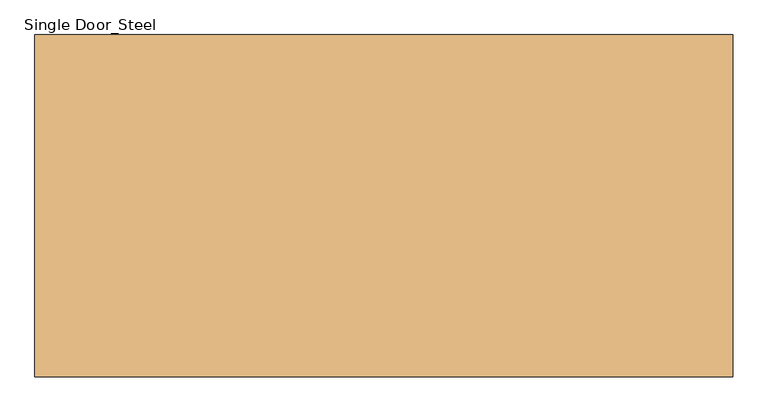
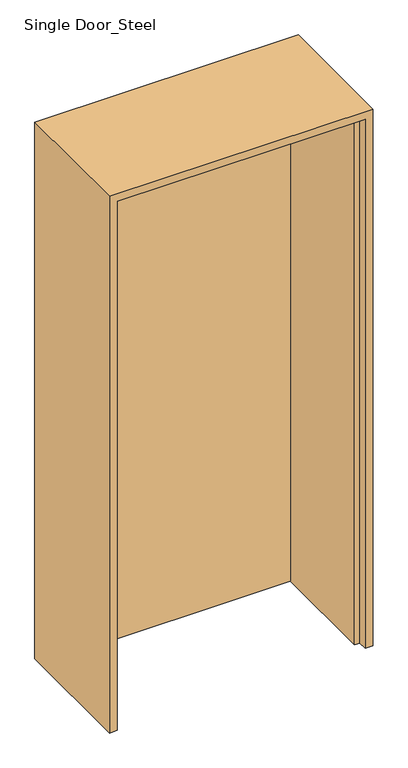
"""IFC4 building model written with IfcOpenShell, lengths in millimetres: door geometry, Single Door_Steel : H_DR_AMB_Single Door_Steel_W1000xH2150."""

from ifc_helpers import new_model, si_unit, origin, origin_with_axes, place, context, project, spatial, polyline, outline, extrude, faceted_brep, source, transform, mapped, element, save


def single_door_steel_7afc0ab2(model_context):
    return source(origin(), model_context, "Body", "SolidModel", [
        extrude(outline(polyline([(470.0, 245.0), (470.0, 210.0), (-470.0, 210.0), (-470.0, 245.0), (470.0, 245.0)])), origin_with_axes(), (0.0, 0.0, 1.0), 2120.0),
        faceted_brep([(470.0, 245.0, 0.0), (500.0, 245.0, 0.0), (500.0, -245.0, 0.0), (470.0, -245.0, 0.0), (470.0, -210.0, 0.0), (450.0, -210.0, 0.0), (450.0, 210.0, 0.0), (470.0, 210.0, 0.0), (470.0, 245.0, 2120.0), (-470.0, 245.0, 2120.0), (-470.0, 245.0, 0.0), (-500.0, 245.0, 0.0), (-500.0, 245.0, 2150.0), (500.0, 245.0, 2150.0), (500.0, -245.0, 2150.0), (-500.0, -245.0, 2150.0), (-500.0, -245.0, 0.0), (-470.0, -245.0, 0.0), (-470.0, -245.0, 2120.0), (470.0, -245.0, 2120.0), (470.0, -210.0, 2120.0), (-470.0, -210.0, 2120.0), (-470.0, -210.0, 0.0), (-450.0, -210.0, 0.0), (-450.0, -210.0, 2100.0), (450.0, -210.0, 2100.0), (450.0, 210.0, 2100.0), (-450.0, 210.0, 2100.0), (-450.0, 210.0, 0.0), (-470.0, 210.0, 0.0), (-470.0, 210.0, 2120.0), (470.0, 210.0, 2120.0)], [[[0, 1, 2, 3, 4, 5, 6, 7]], [[1, 0, 8, 9, 10, 11, 12, 13]], [[2, 1, 13, 14]], [[3, 2, 14, 15, 16, 17, 18, 19]], [[4, 3, 19, 20]], [[5, 4, 20, 21, 22, 23, 24, 25]], [[6, 5, 25, 26]], [[7, 6, 26, 27, 28, 29, 30, 31]], [[0, 7, 31, 8]], [[9, 30, 29, 10]], [[10, 29, 28, 23, 22, 17, 16, 11]], [[15, 12, 11, 16]], [[21, 18, 17, 22]], [[27, 24, 23, 28]], [[14, 13, 12, 15]], [[20, 19, 18, 21]], [[26, 25, 24, 27]], [[8, 31, 30, 9]]]),
    ])


if __name__ == "__main__":
    model = new_model("IFC4")
    model_context = context("Model", 3, world=origin())
    ifc_project = project(units=[si_unit("LENGTHUNIT", "METRE", prefix="MILLI")], contexts=[model_context])
    site = spatial("IfcSite", under=ifc_project)
    building = spatial("IfcBuilding", under=site)
    placement = place(None, origin())
    single_door_steel_shape = single_door_steel_7afc0ab2(model_context)
    element("IfcDoor", 1, ObjectType="Single Door_Steel : H_DR_AMB_Single Door_Steel_W1000xH2150", at=placement, inside=building, context=model_context, shape_type="MappedRepresentation", body=[
        mapped(single_door_steel_shape, transform((0.0, 0.0, 0.0), x_axis=(1.0, 0.0, 0.0), y_axis=(0.0, 1.0, 0.0), z_axis=(0.0, 0.0, 1.0))),
    ])
    save(model, "model.ifc")

# Revit data of these elements
# Type "Single Door_Steel : H_DR_AMB_Single Door_Steel_W1000xH2150"
#   Type Mark = "364"
#   Analytic Construction = "<None>"
#   프레임 투영 외부. = 25.000 mm
#   프레임 투영 내부. = 25.000 mm
#   프레임 폭 = 75.000 mm
#   Height = 2150.000 mm
#   Width = 1000.000 mm
#   Define Thermal Properties by = 1
#   문 패널 = none
#   문 프레임 = none
#   Function = (empty or 0)
#   Wall Closure = (empty or 0)
